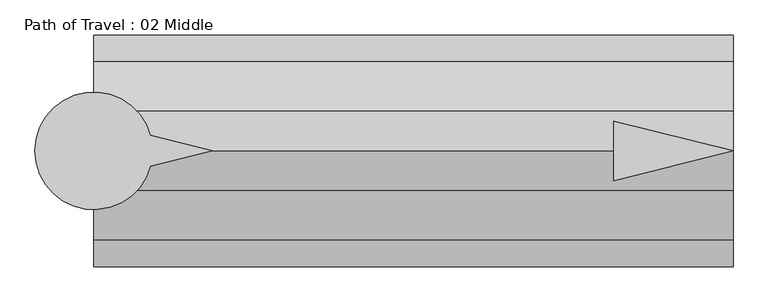
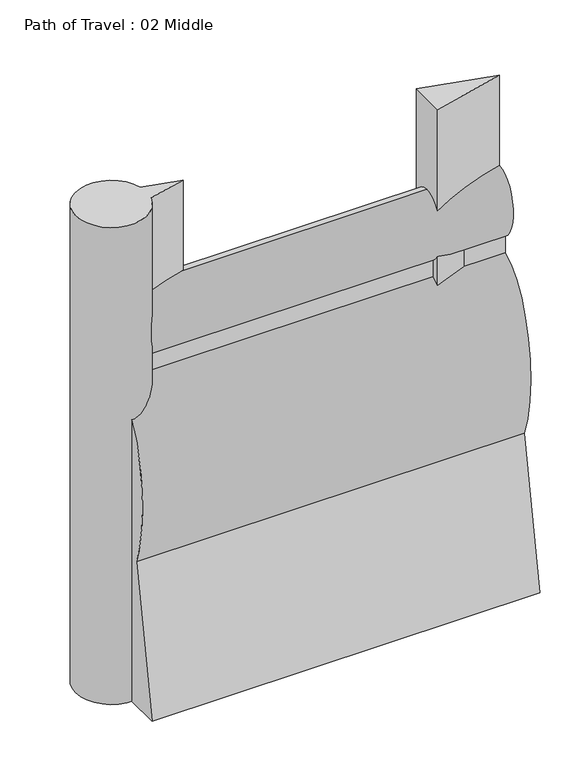
"""IFC4 building model written with IfcOpenShell, lengths in millimetres: proxy geometry, Path of Travel : 02 Middle."""

from ifc_helpers import new_model, si_unit, point, frame, frame_2d, origin, origin_with_axes, place, context, project, spatial, polyline, circle_curve, ellipse_curve, trimmed, segment, composite_curve, outline, extrude, source, transform, mapped, element, save
from ifc_brep_helpers import plane_surface, extruded_surface, advanced_brep


def path_of_travel_02_middle_f1598f8f(model_context):
    return source(origin(), model_context, "Body", "SolidModel", [
        advanced_brep(
        [(227.5554837, 0.0, 1727.2), (227.5554837, 42.9018657, 1436.6534209), (227.5554837, 42.9018657, 1363.4763406), (227.5554837, 184.1186263, 643.4144547), (227.5554837, 297.5699544, 0.0), (227.5554837, 145.6574193, 0.0), (227.5554837, 0.0, 584.2), (227.5554837, -145.6574193, 0.0), (227.5554837, -297.5699544, 0.0), (227.5554837, -184.1186263, 643.4144547), (227.5554837, -42.9018657, 1363.4763406), (227.5554837, -42.9018657, 1436.6534209), (1868.1926692, 0.0, 1727.2), (1868.1926692, -42.9018657, 1436.6534209), (1868.1926692, -42.9018657, 1363.4763406), (1868.1926692, -184.1186263, 643.4144547), (1868.1926692, -297.5699544, 0.0), (1868.1926692, -145.6574193, 0.0), (1868.1926692, 0.0, 584.2), (1868.1926692, 145.6574193, 0.0), (1868.1926692, 297.5699544, 0.0), (1868.1926692, 184.1186263, 643.4144547), (1868.1926692, 42.9018657, 1363.4763406), (1868.1926692, 42.9018657, 1436.6534209)],
        [
            (0, 1, ellipse_curve(frame((227.5554837, 0.0, 1574.8), z_axis=(-1.0, 0.0, 0.0), x_axis=(0.0, 0.0, 1.0)), 152.4, 101.6)),
            (1, 2),
            (2, 3, ellipse_curve(frame((227.5554837, 0.0, 914.4), z_axis=(-1.0, 0.0, 0.0), x_axis=(0.0, 0.0, -1.0)), 457.2, 228.6)),
            (3, 4),
            (4, 5),
            (5, 6),
            (6, 7),
            (7, 8),
            (8, 9),
            (9, 10, ellipse_curve(frame((227.5554837, 0.0, 914.4), z_axis=(-1.0, 0.0, 0.0), x_axis=(0.0, 0.0, -1.0)), 457.2, 228.6)),
            (10, 11),
            (11, 0, ellipse_curve(frame((227.5554837, 0.0, 1574.8), z_axis=(-1.0, 0.0, 0.0), x_axis=(0.0, 0.0, 1.0)), 152.4, 101.6)),
            (12, 13, ellipse_curve(frame((1868.1926692, 0.0, 1574.8), z_axis=(1.0, 0.0, 0.0), x_axis=(0.0, 0.0, 1.0)), 152.4, 101.6)),
            (13, 14),
            (14, 15, ellipse_curve(frame((1868.1926692, 0.0, 914.4), z_axis=(1.0, 0.0, 0.0), x_axis=(0.0, 0.0, -1.0)), 457.2, 228.6)),
            (15, 16),
            (16, 17),
            (17, 18),
            (18, 19),
            (19, 20),
            (20, 21),
            (21, 22, ellipse_curve(frame((1868.1926692, 0.0, 914.4), z_axis=(1.0, 0.0, 0.0), x_axis=(0.0, 0.0, -1.0)), 457.2, 228.6)),
            (22, 23),
            (23, 12, ellipse_curve(frame((1868.1926692, 0.0, 1574.8), z_axis=(1.0, 0.0, 0.0), x_axis=(0.0, 0.0, 1.0)), 152.4, 101.6)),
            (0, 12),
            (23, 1),
            (22, 2),
            (21, 3),
            (20, 4),
            (19, 5),
            (18, 6),
            (17, 7),
            (16, 8),
            (15, 9),
            (14, 10),
            (13, 11),
        ],
        [
            plane_surface(frame((227.5554837, 0.0, 0.0), z_axis=(-1.0, 0.0, 0.0), x_axis=(0.0, 0.0, 1.0))),
            plane_surface(frame((1868.1926692, 0.0, 0.0), z_axis=(1.0, 0.0, 0.0), x_axis=(0.0, 0.0, 1.0))),
            extruded_surface(trimmed(ellipse_curve(frame((1868.1926692, 0.0, 1574.8), z_axis=(-1.0, 0.0, 0.0), x_axis=(0.0, 0.0, 1.0)), 152.4, 101.6), [point((1868.1926692, 0.0, 1727.2))], [point((1868.1926692, 42.9018657, 1436.6534209))], True, "CARTESIAN"), (-1640.6371855, 0.0, 0.0), 1640.6371855),
            plane_surface(frame((227.5554837, 42.9018657, 1436.6534209), z_axis=(0.0, 1.0, 0.0), x_axis=(1.0, 0.0, 0.0))),
            extruded_surface(trimmed(ellipse_curve(frame((1868.1926692, 0.0, 914.4), z_axis=(-1.0, 0.0, 0.0), x_axis=(0.0, 0.0, -1.0)), 457.2, 228.6), [point((1868.1926692, 42.9018657, 1363.4763406))], [point((1868.1926692, 184.1186263, 643.4144547))], True, "CARTESIAN"), (-1640.6371855, 0.0, 0.0), 1640.6371855),
            plane_surface(frame((227.5554837, 184.1186263, 643.4144547), z_axis=(0.0, 0.9848077530122078, 0.1736481776669322), x_axis=(1.0, 0.0, 0.0))),
            plane_surface(frame((227.5554837, 297.5699544, 0.0), z_axis=(0.0, 0.0, -1.0), x_axis=(1.0, 0.0, 0.0))),
            plane_surface(frame((227.5554837, 145.6574193, 0.0), z_axis=(0.0, -0.9702957262760199, -0.2419218955995739), x_axis=(1.0, 0.0, 0.0))),
            plane_surface(frame((227.5554837, 0.0, 584.2), z_axis=(0.0, 0.9702957262759961, -0.24192189559966923), x_axis=(1.0, 0.0, 0.0))),
            plane_surface(frame((227.5554837, -145.6574193, 0.0), z_axis=(0.0, 0.0, -1.0), x_axis=(1.0, 0.0, 0.0))),
            plane_surface(frame((227.5554837, -297.5699544, 0.0), z_axis=(0.0, -0.984807753012208, 0.17364817766693066), x_axis=(1.0, 0.0, 0.0))),
            extruded_surface(trimmed(ellipse_curve(frame((1868.1926692, 0.0, 914.4), z_axis=(-1.0, 0.0, 0.0), x_axis=(0.0, 0.0, -1.0)), 457.2, 228.6), [point((1868.1926692, -184.1186263, 643.4144547))], [point((1868.1926692, -42.9018657, 1363.4763406))], True, "CARTESIAN"), (-1640.6371855, 0.0, 0.0), 1640.6371855),
            plane_surface(frame((227.5554837, -42.9018657, 1363.4763406), z_axis=(0.0, -1.0, 0.0), x_axis=(1.0, 0.0, 0.0))),
            extruded_surface(trimmed(ellipse_curve(frame((1868.1926692, 0.0, 1574.8), z_axis=(-1.0, 0.0, 0.0), x_axis=(0.0, 0.0, 1.0)), 152.4, 101.6), [point((1868.1926692, -42.9018657, 1436.6534209))], [point((1868.1926692, 0.0, 1727.2))], True, "CARTESIAN"), (-1640.6371855, 0.0, 0.0), 1640.6371855),
        ],
        [
            (0, [[1, 2, 3, 4, 5, 6, 7, 8, 9, 10, 11, 12]]),
            (1, [[13, 14, 15, 16, 17, 18, 19, 20, 21, 22, 23, 24]]),
            (2, [[-1, 25, -24, 26]]),
            (3, [[-2, -26, -23, 27]]),
            (4, [[-3, -27, -22, 28]]),
            (5, [[-4, -28, -21, 29]]),
            (6, [[-5, -29, -20, 30]]),
            (7, [[-6, -30, -19, 31]]),
            (8, [[-7, -31, -18, 32]]),
            (9, [[-8, -32, -17, 33]]),
            (10, [[-9, -33, -16, 34]]),
            (11, [[-10, -34, -15, 35]]),
            (12, [[-11, -35, -14, 36]]),
            (13, [[-12, -36, -13, -25]]),
        ],
    ),
        extrude(outline(polyline([(1562.1875227, 76.2006338), (1868.1926692, 0.0), (1562.1875227, -76.2006338), (1562.1875227, 76.2006338)])), origin_with_axes(), (0.0, 0.0, 1.0), 2129.5973753),
        extrude(outline(composite_curve([segment(polyline([(372.7837828, 39.4440225), (531.182385, 0.0), (372.7837828, -39.4440225)]), True, "CONTINUOUS"), segment(trimmed(circle_curve(frame_2d((227.2200886, 0.0)), 150.8131956), [point((372.7837828, -39.4440225))], [point((372.7837828, 39.4440225))], False, "CARTESIAN"), True, "CONTINUOUS")], self_intersect=False)), origin_with_axes(), (0.0, 0.0, 1.0), 2129.5973753),
    ])


if __name__ == "__main__":
    model = new_model("IFC4")
    model_context = context("Model", 3, world=origin())
    ifc_project = project(units=[si_unit("LENGTHUNIT", "METRE", prefix="MILLI")], contexts=[model_context])
    site = spatial("IfcSite", under=ifc_project)
    building = spatial("IfcBuilding", under=site)
    placement = place(None, origin())
    path_of_travel_02_middle_shape = path_of_travel_02_middle_f1598f8f(model_context)
    element("IfcBuildingElementProxy", 1, Name="Path of Travel : 02 Middle", ObjectType="Path of Travel : 02 Middle", at=placement, inside=building, context=model_context, shape_type="MappedRepresentation", body=[
        mapped(path_of_travel_02_middle_shape, transform((0.0, 0.0, 0.0), x_axis=(1.0, 0.0, 0.0), y_axis=(0.0, 1.0, 0.0), z_axis=(0.0, 0.0, 1.0))),
    ])
    save(model, "model.ifc")

# Revit data of these elements
# Type "Path of Travel : 02 Middle"
#   Path of Egress [instance default] = 4' - 0"
#   built-in parameter 1001306 [instance default] = 4 (stored number, unit not read)
#   Dot at Start = no
#   Arrow in Middle = yes
#   Arrow at End = no
#   Egress Path = none
# Element 1 (IfcBuildingElementProxy, "Path of Travel : 02 Middle")
#   Path of Egress = 5' - 4.59202"
#   built-in parameter 1001306 = 5.38267 (stored number, unit not read)
#   Materials on its faces: "Egress Path Solid", "solid"
# Materials
#   "Egress Path Solid": class "Unassigned", colour RGB 255 128 64, transparency 0.75, Comments = "Rendering appearance not upgraded "
#   "solid": class "Generic", colour RGB 120 120 120, transparency 0, Cost = 0
